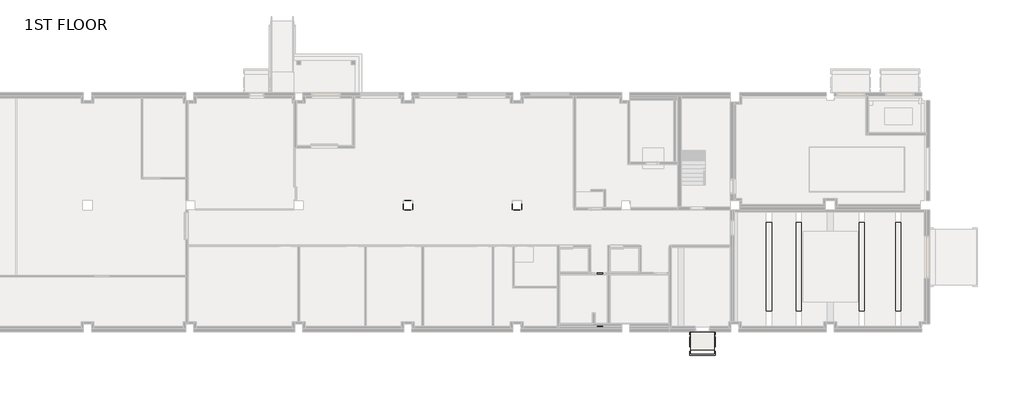
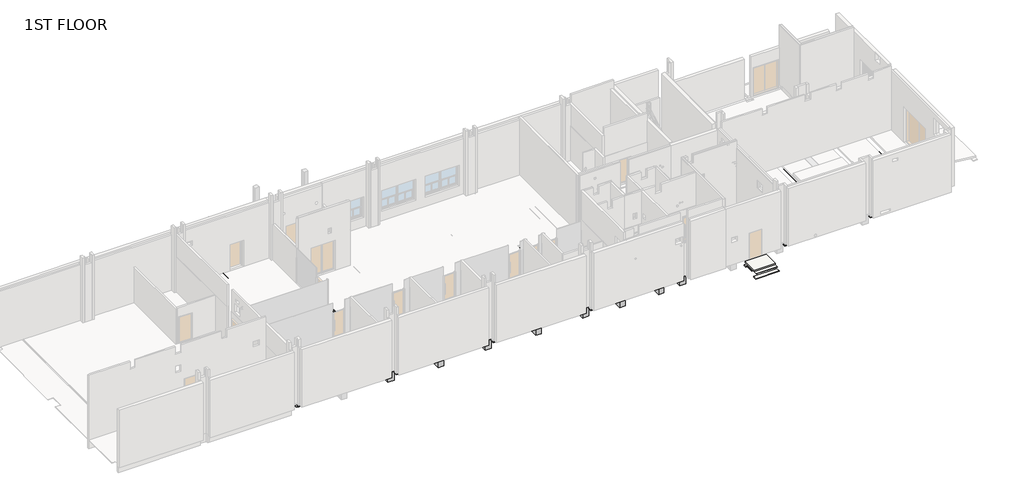
# One storey, part 9 of 15: 19 beams, 7 slabs.
# Revit data of these elements (continued)
# Type "RC Beam_Rectangular : H_SB_AR S16_TG-UG_450x800_1B1B" (continued)
#   중앙부 보조근 = ""
#   중앙부 늑근 = ""
#   외단부 하부근 = ""
#   외단부 상부근 = ""
#   외단부 보조근 = ""
#   외단부 늑근 = ""
#   부호 = "TG3"
#   내단부 하부근 = ""
#   내단부 상부근 = ""
#   내단부 보조근 = ""
#   내단부 늑근 = ""
#   ALL 하부근 = "3-D20"
#   ALL 상부근 = "3-D20"
#   ALL 보조근 = ""
#   ALL 늑근 = "2-D10 @120"
#   H_Rebar Ratio = 0.14
#   Width = 450 mm
#   Height = 800 mm
#   Length [instance default] = 1524 mm
#   b = 450 mm
#   h = 800 mm
#   hec_material3 [instance default] = none
#   hec_material2 [instance default] = none
#   hec_material1 [instance default] = none
#   Structural Material [instance default] = none
#   Assembly Code = ""
# Type "H_SF_AR_B08_Stoop_T150"
#   Type Comments = "CV-AG"
#   H_Rebar Ratio = 0.1
#   Layers, outside or top first: 150 mm "Concrete_f'c=28MPa(Cylender)" (function 1)
# Type "H_SF_AR_B08_Stoop_T125"
#   Type Comments = "CV-AG"
#   H_Rebar Ratio = 0.1
#   Layers, outside or top first: 125 mm "Concrete_f'c=28MPa(Cylender)" (function 1)
# Type "H_SF_AR_S18_Lean_T50"
#   Type Comments = "Lean"
#   Layers, outside or top first: 50 mm "Concrete_f'c=14MPa(Cylender)" (function 1)
# Elements 1, 2, 3, 4 (IfcBeam, "RC Beam_Rectangular : H_SB_AR S16_TG-UG_500x800_1G2")
#   Comments = ""
#   hec_material3 = none
#   hec_material2 = none
#   hec_material1 = none
#   Structural Material = Concrete_f'c=28MPa(Cylender)
#   Phase Created = New Construction
#   Materials on its faces: "Concrete_f'c=28MPa(Cylender)"
# Elements 5, 7, 10, 11, 12 (IfcBeam, "RC Beam_Rectangular : H_SB_AR S16_TG-UG_500x800_1G1")
#   Comments = ""
#   hec_material3 = none
#   hec_material2 = none
#   hec_material1 = none
#   Structural Material = Concrete_f'c=28MPa(Cylender)
#   Phase Created = New Construction
#   Materials on its faces: "Concrete_f'c=28MPa(Cylender)"
# Elements 6, 8, 9 (IfcBeam, "RC Beam_Rectangular : H_SB_AR S16_TG-UG_450x800_1B1")
#   Comments = ""
#   hec_material3 = none
#   hec_material2 = none
#   hec_material1 = none
#   Structural Material = Concrete_f'c=28MPa(Cylender)
#   Phase Created = New Construction
#   Materials on its faces: "Concrete_f'c=28MPa(Cylender)"
# Elements 13, 14, 15 (IfcBeam, "RC Beam_Rectangular : H_SB_AR S16_TG-UG_450x800_1B1A")
#   Comments = ""
#   hec_material3 = none
#   hec_material2 = none
#   hec_material1 = none
#   Structural Material = Concrete_f'c=28MPa(Cylender)
#   Phase Created = New Construction
#   Materials on its faces: "Concrete_f'c=28MPa(Cylender)"
# Element 16 (IfcBeam, "RC Beam_Rectangular : H_SB_AR S16_TG-UG_450x700_1B1B")
#   Comments = ""
#   hec_material3 = none
#   hec_material2 = none
#   hec_material1 = none
#   Structural Material = Concrete_f'c=28MPa(Cylender)
#   Phase Created = New Construction
#   Materials on its faces: "Concrete_f'c=28MPa(Cylender)"
# Element 17 (IfcBeam, "RC Beam_Rectangular : H_SB_AR S16_TG-UG_500x700_1G1A")
#   Comments = ""
#   hec_material3 = none
#   hec_material2 = none
#   hec_material1 = none
#   Structural Material = Concrete_f'c=28MPa(Cylender)
#   Phase Created = New Construction
#   Materials on its faces: "Concrete_f'c=28MPa(Cylender)"
# Element 18 (IfcBeam, "RC Beam_Rectangular : H_SB_AR S16_TG-UG_500x800_1G1A")
#   IfcGUID = "1eK$f4e8T3POk8TBv2woV1"
#   Comments = ""
#   hec_material3 = none
#   hec_material2 = none
#   hec_material1 = none
#   Structural Material = Concrete_f'c=28MPa(Cylender)
#   Phase Created = New Construction
#   Materials on its faces: "Concrete_f'c=28MPa(Cylender)"
# Element 19 (IfcBeam, "RC Beam_Rectangular : H_SB_AR S16_TG-UG_450x800_1B1B")
#   IfcGUID = "1eK$f4e8T3POk8TBv2woGm"
#   Comments = ""
#   hec_material3 = none
#   hec_material2 = none
#   hec_material1 = none
#   Structural Material = Concrete_f'c=28MPa(Cylender)
#   Phase Created = New Construction
#   Materials on its faces: "Concrete_f'c=28MPa(Cylender)"
# Element 20 (IfcSlab, "H_SF_AR_B08_Stoop_T150")
#   Comments = ""
#   built-in parameter 1001955 = -3.14159 (stored number, unit not read)
#   Height Offset From Level = -50 mm
#   built-in parameter 1001954 = 1
#   Phase Created = New Construction
#   Materials on its faces: "Concrete_f'c=28MPa(Cylender)"
# Element 21 (IfcSlab, "H_SF_AR_B08_Stoop_T125")
#   Comments = ""
#   built-in parameter 1001955 = -3.14159 (stored number, unit not read)
#   Height Offset From Level = -175 mm
#   built-in parameter 1001954 = 1
#   Phase Created = New Construction
#   Materials on its faces: "Concrete_f'c=28MPa(Cylender)"
# Element 22 (IfcSlab, "H_SF_AR_S18_Lean_T50")
#   Comments = ""
#   built-in parameter 1001955 = -3.14159 (stored number, unit not read)
#   Height Offset From Level = -500 mm
#   built-in parameter 1001954 = 1
#   Phase Created = New Construction
#   Materials on its faces: "Concrete_f'c=14MPa(Cylender)"
# Element 23 (IfcSlab, "H_SF_AR_S18_Lean_T50")
#   Comments = ""
#   built-in parameter 1001955 = -3.14159 (stored number, unit not read)
#   Height Offset From Level = -350 mm
#   built-in parameter 1001954 = 1
#   Phase Created = New Construction
#   Materials on its faces: "Concrete_f'c=14MPa(Cylender)"
# Element 24 (IfcSlab, "H_SF_AR_S18_Lean_T50")
#   Comments = ""
#   built-in parameter 1001955 = -3.14159 (stored number, unit not read)
#   Height Offset From Level = -200 mm
#   built-in parameter 1001954 = 1
#   Phase Created = New Construction
#   Materials on its faces: "Concrete_f'c=14MPa(Cylender)"
# Element 25 (IfcSlab, "H_SF_AR_S18_Lean_T50")
#   Comments = ""
#   Height Offset From Level = -910 mm
#   built-in parameter 1001954 = 1
#   Phase Created = New Construction
#   Materials on its faces: "Concrete_f'c=14MPa(Cylender)"
# Element 26 (IfcSlab, "H_SF_AR_S18_Lean_T50")
#   Comments = ""
#   Height Offset From Level = -260 mm
#   built-in parameter 1001954 = 1
#   Phase Created = New Construction
#   Materials on its faces: "Concrete_f'c=14MPa(Cylender)"
# Materials
#   "Concrete_f'c=28MPa(Cylender)": class "Concrete", colour RGB 176 176 176, transparency 0, Description = "Reinf. Conc.", Cost = 0, Image = Concrete.Cast-In-Place.Flat.Polished.Grey.jpg
#   "Concrete_f'c=14MPa(Cylender)": class "Concrete", colour RGB 177 177 177, transparency 0, Description = "Reinf. Conc.", Cost = 0
